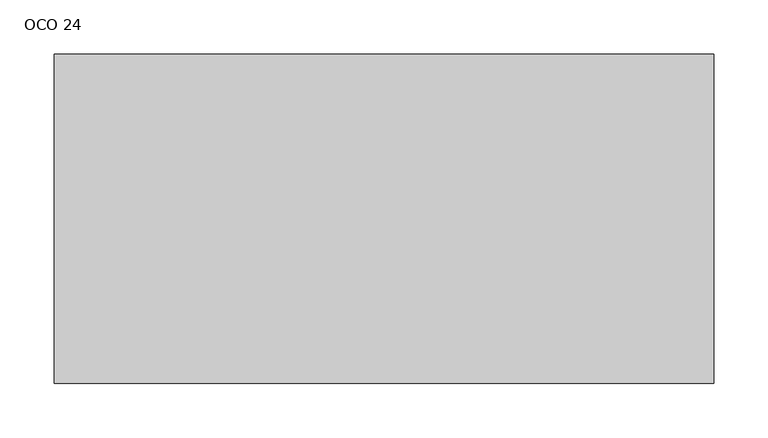
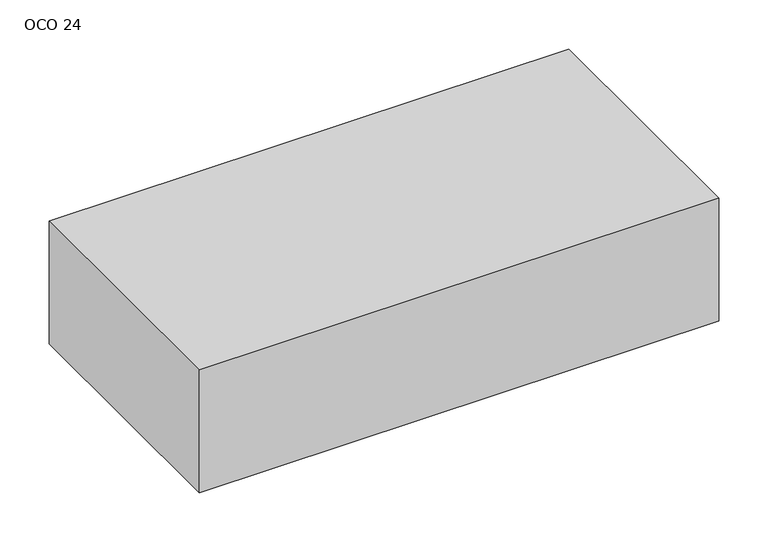
"""IFC4 building model written with IfcOpenShell, lengths in millimetres: furniture geometry, Accessories-Merillat-Wall-Open_Cube_Organizer : OCO 24."""

from ifc_helpers import new_model, si_unit, frame, origin, place, context, project, spatial, polyline, outline, extrude, faceted_brep, source, transform, mapped, element, save


def oco_24_403fa207(model_context):
    return source(origin(), model_context, "Body", "SolidModel", [
        extrude(outline(polyline([(-75.0038372, 364.8986578), (-62.3038372, 364.8986578), (-62.3038372, 80.9112557), (-75.0038372, 80.9112557), (-75.0038372, 364.8986578)])), frame((0.0, 0.0, 1990.725), z_axis=(0.0, 0.0, 1.0), x_axis=(1.0, 0.0, 0.0)), (0.0, 0.0, 1.0), 133.35),
        extrude(outline(polyline([(121.8461628, 364.8986578), (134.5461628, 364.8986578), (134.5461628, 80.9112557), (121.8461628, 80.9112557), (121.8461628, 364.8986578)])), frame((0.0, 0.0, 1990.725), z_axis=(0.0, 0.0, 1.0), x_axis=(1.0, 0.0, 0.0)), (0.0, 0.0, 1.0), 133.35),
        extrude(outline(polyline([(-271.8538372, 364.8986578), (-259.1538372, 364.8986578), (-259.1538372, 80.9112557), (-271.8538372, 80.9112557), (-271.8538372, 364.8986578)])), frame((0.0, 0.0, 1990.725), z_axis=(0.0, 0.0, 1.0), x_axis=(1.0, 0.0, 0.0)), (0.0, 0.0, 1.0), 133.35),
        extrude(outline(polyline([(318.6961628, 364.8986578), (331.3961628, 364.8986578), (331.3961628, 80.9112557), (318.6961628, 80.9112557), (318.6961628, 364.8986578)])), frame((0.0, 0.0, 1990.725), z_axis=(0.0, 0.0, 1.0), x_axis=(1.0, 0.0, 0.0)), (0.0, 0.0, 1.0), 133.35),
        faceted_brep([(334.5711628, 366.7125, 1981.2), (-275.0288372, 366.7125, 1981.2), (-275.0288372, 366.7125, 2133.6), (334.5711628, 366.7125, 2133.6), (318.6961628, 366.7125, 1990.725), (318.6961628, 366.7125, 2124.075), (-259.1538372, 366.7125, 2124.075), (-259.1538372, 366.7125, 1990.725), (334.5711628, 61.9125, 1981.2), (334.5711628, 61.9125, 2133.6), (-275.0288372, 61.9125, 2133.6), (-275.0288372, 61.9125, 1981.2), (318.6961628, 80.9112557, 1990.725), (-259.1538372, 80.9112557, 1990.725), (-259.1538372, 80.9112557, 2124.075), (318.6961628, 80.9112557, 2124.075)], [[[0, 1, 2, 3], [4, 5, 6, 7]], [[8, 9, 10, 11]], [[1, 0, 8, 11]], [[2, 1, 11, 10]], [[3, 2, 10, 9]], [[0, 3, 9, 8]], [[12, 13, 14, 15]], [[12, 15, 5, 4]], [[15, 14, 6, 5]], [[14, 13, 7, 6]], [[13, 12, 4, 7]]]),
    ])


if __name__ == "__main__":
    model = new_model("IFC4")
    model_context = context("Model", 3, world=origin())
    ifc_project = project(units=[si_unit("LENGTHUNIT", "METRE", prefix="MILLI")], contexts=[model_context])
    site = spatial("IfcSite", under=ifc_project)
    building = spatial("IfcBuilding", under=site)
    placement = place(None, origin())
    oco_24_shape = oco_24_403fa207(model_context)
    element("IfcFurniture", 1, ObjectType="Accessories-Merillat-Wall-Open_Cube_Organizer : OCO 24", at=placement, inside=building, context=model_context, shape_type="MappedRepresentation", body=[
        mapped(oco_24_shape, transform((0.0, 0.0, 0.0), x_axis=(1.0, 0.0, 0.0), y_axis=(0.0, 1.0, 0.0), z_axis=(0.0, 0.0, 1.0))),
    ])
    save(model, "model.ifc")

# Revit data of these elements
# Type "Accessories-Merillat-Wall-Open_Cube_Organizer : OCO 24"
#   URL = "https://www.merillat.com/"
#   Product Page URL = "https://www.merillat.com/our-products/rooms/kitchen/"
#   Product Documentation Link = "http://merillatbusiness.com/wp-content/uploads/2014/07/Merillat_Classic_Catalog.pdf"
#   Model = "OCO18"
#   Manufacturer = "Merillat"
#   Finish = "Wood"
#   Description = "Open Cube Organizer 3 compartments"
#   Construction Type = "Wall Cabinet"
#   Assembly Code = "C1030410"
#   Depth = 1' - 0"
#   Height = 0' - 6"
#   Top Of Cabinet = 7' - 0"
#   Width = 2' - 0"
#   COBie.Type = no
#   Number of Compartments = 3
#   Actual Number of Compartments = 4
#   Cabinet Material = Wood - Merillat - Pecan(1)
# Element 1 (IfcFurniture, "Accessories-Merillat-Wall-Open_Cube_Organizer : OCO 24")
#   Materials on its faces: "Wood - Merillat - Pecan(1)"
# Materials
#   "Wood - Merillat - Pecan(1)": class "Wood", colour RGB 108 67 43, transparency 0, Cost = 0
